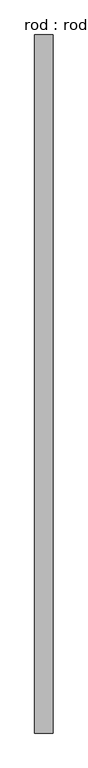
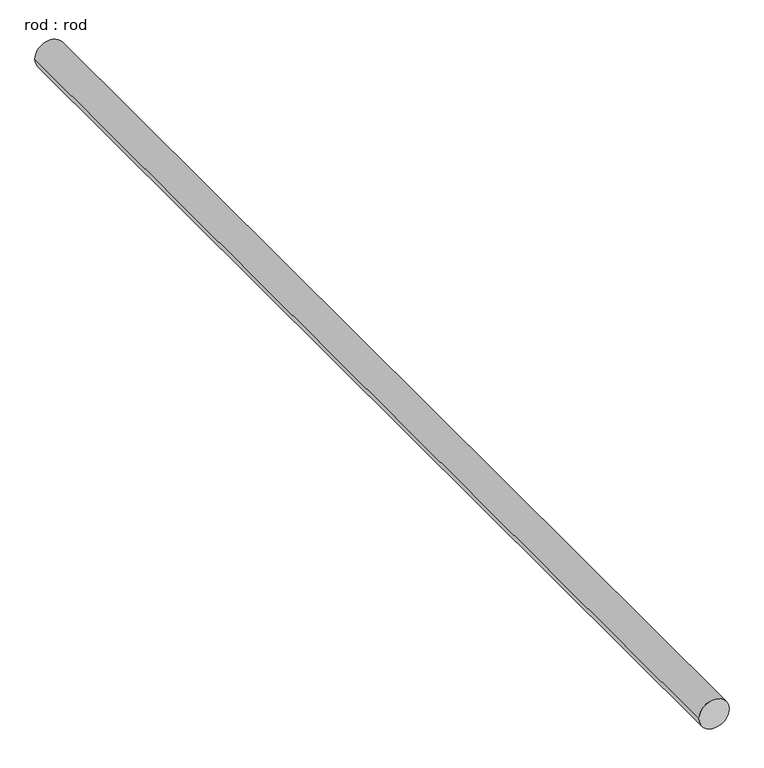
"""IFC4 building model written with IfcOpenShell, lengths in millimetres: proxy geometry, rod : rod."""

from ifc_helpers import new_model, si_unit, point, frame, frame_2d, origin, place, context, project, spatial, circle_curve, trimmed, segment, composite_curve, outline, extrude, source, transform, mapped, element, save


def rod_rod_c5d1c320(model_context):
    return source(origin(), model_context, "Body", "SweptSolid", [
        extrude(outline(composite_curve([segment(trimmed(circle_curve(frame_2d((0.0108462, 0.0)), 200.0), [point((0.0108462, 200.0))], [point((0.0108462, -200.0))], False, "CARTESIAN"), True, "CONTINUOUS"), segment(trimmed(circle_curve(frame_2d((0.0108462, 0.0)), 200.0), [point((0.0108462, -200.0))], [point((0.0108462, 200.0))], False, "CARTESIAN"), True, "CONTINUOUS")], self_intersect=False)), frame((0.0, -3522.6691295, 0.0), z_axis=(0.0, 1.0, 0.0), x_axis=(0.0, 0.0, 1.0)), (0.0, 0.0, 1.0), 15230.7954897),
    ])


if __name__ == "__main__":
    model = new_model("IFC4")
    model_context = context("Model", 3, world=origin())
    ifc_project = project(units=[si_unit("LENGTHUNIT", "METRE", prefix="MILLI")], contexts=[model_context])
    site = spatial("IfcSite", under=ifc_project)
    building = spatial("IfcBuilding", under=site)
    placement = place(None, origin())
    rod_rod_shape = rod_rod_c5d1c320(model_context)
    element("IfcBuildingElementProxy", 1, Name="rod : rod", ObjectType="rod : rod", at=placement, inside=building, context=model_context, shape_type="MappedRepresentation", body=[
        mapped(rod_rod_shape, transform((0.0, 0.0, 0.0), x_axis=(1.0, 0.0, 0.0), y_axis=(0.0, 1.0, 0.0), z_axis=(0.0, 0.0, 1.0))),
    ])
    save(model, "model.ifc")

# Revit data of these elements
# Type "rod : rod"
#   Default Elevation = 0
